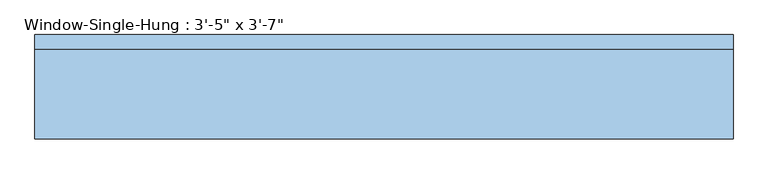
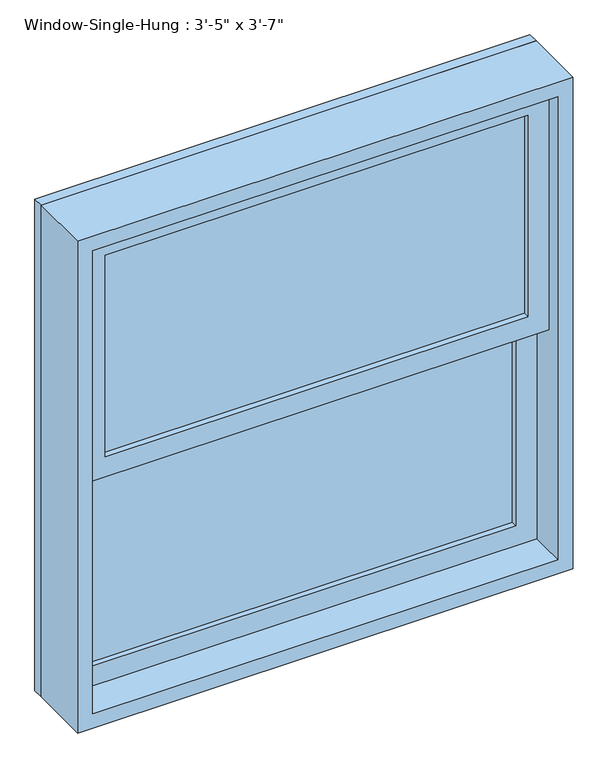
"""IFC4 building model written with IfcOpenShell, lengths in millimetres: window geometry."""

import ifcopenshell
import ifcopenshell.guid

model = None  # the IFC model being written
_history = None  # IfcOwnerHistory: only IFC2X3 demands one
_inside = {}  # id of a spatial element -> (the spatial element, [elements in it])
_under = {}  # id of a project, library or spatial element -> (it, [spatial elements below it])
_declared = {}  # id of a project -> (the project, [libraries it declares])
_typed = {}  # id of a type object -> (the type object, [elements of that type])
_made_of = {}  # id of a material, layer set ... -> (it, [elements and type objects made of it])


def new_model(schema):
    """Start an empty IFC model of exactly this schema.

    Asked for "IFC4X3", IfcOpenShell would pick the latest addendum, in which some entities
    have other attributes; the version numbers below select the first issue.
    IFC2X3 requires an IfcOwnerHistory on every rooted entity: one is made here for all.
    """
    global model, _history
    if schema == "IFC4X3":
        model = ifcopenshell.file(schema_version=(4, 3, 0, 0))
    else:
        model = ifcopenshell.file(schema=schema)
    _inside.clear()
    _under.clear()
    _declared.clear()
    _typed.clear()
    _made_of.clear()
    _history = None
    if model.schema == "IFC2X3":
        org = make("IfcOrganization", Name="unknown")
        user = make(
            "IfcPersonAndOrganization",
            ThePerson=make("IfcPerson", FamilyName="unknown"),
            TheOrganization=org,
        )
        app = make(
            "IfcApplication",
            ApplicationDeveloper=org,
            Version="unknown",
            ApplicationFullName="unknown",
            ApplicationIdentifier="unknown",
        )
        _history = make(
            "IfcOwnerHistory",
            OwningUser=user,
            OwningApplication=app,
            ChangeAction="ADDED",
            CreationDate=0,
        )
    return model


def make(cls, **values):
    """One entity of the class cls with the attributes given. An attribute that is None is left unset."""
    return model.create_entity(
        cls, **{name: value for name, value in values.items() if value is not None}
    )


def rooted(cls, **values):
    """An entity with a GlobalId (a new one), such as an element, a storey or a relation."""
    return make(cls, GlobalId=ifcopenshell.guid.new(), OwnerHistory=_history, **values)


def si_unit(unit_type, name, prefix=None):
    """IfcSIUnit, for example si_unit("LENGTHUNIT", "METRE", prefix="MILLI")."""
    return make("IfcSIUnit", UnitType=unit_type, Prefix=prefix, Name=name)


def assignment(units):
    """IfcUnitAssignment: the units of a project."""
    return None if units is None else make("IfcUnitAssignment", Units=units)


def point(xyz):
    """IfcCartesianPoint."""
    return None if xyz is None else make("IfcCartesianPoint", Coordinates=xyz)


def direction(xyz):
    """IfcDirection."""
    return None if xyz is None else make("IfcDirection", DirectionRatios=xyz)


def frame(location, z_axis=None, x_axis=None):
    """IfcAxis2Placement3D, a coordinate frame: its origin and axes. An axis left out is left unset."""
    return make(
        "IfcAxis2Placement3D",
        Location=point(location),
        Axis=direction(z_axis),
        RefDirection=direction(x_axis),
    )


def origin():
    """The frame at (0, 0, 0) with its axes left unset."""
    return frame((0.0, 0.0, 0.0))


def place(relative_to, where):
    """IfcLocalPlacement: puts the frame where relative to a parent placement (None: the world)."""
    return make(
        "IfcLocalPlacement", PlacementRelTo=relative_to, RelativePlacement=where
    )


def context(
    kind, dimensions, precision=None, world=None, true_north=None, identifier=None
):
    """IfcGeometricRepresentationContext, for example the 3D "Model" context."""
    return make(
        "IfcGeometricRepresentationContext",
        ContextIdentifier=identifier,
        ContextType=kind,
        CoordinateSpaceDimension=dimensions,
        Precision=precision,
        WorldCoordinateSystem=world,
        TrueNorth=true_north,
    )


def project(units=None, contexts=None):
    """IfcProject with its units and contexts."""
    return rooted(
        "IfcProject",
        Name="project",
        RepresentationContexts=contexts,
        UnitsInContext=assignment(units),
    )


def spatial(cls, under=None, at=None, **own):
    """A site, building, storey or space (cls), placed at a placement, below another one or the project."""
    s = rooted(cls, ObjectPlacement=at, **own)
    if under is not None:
        _under.setdefault(under.id(), (under, []))[1].append(s)
    return s


def polyline(points):
    """IfcPolyline through the points."""
    return make("IfcPolyline", Points=[point(p) for p in points])


def outline(outer, holes=None, kind="AREA"):
    """IfcArbitraryClosedProfileDef: a profile drawn as a closed curve; with holes, ...WithVoids."""
    if holes is None:
        return make("IfcArbitraryClosedProfileDef", ProfileType=kind, OuterCurve=outer)
    return make(
        "IfcArbitraryProfileDefWithVoids",
        ProfileType=kind,
        OuterCurve=outer,
        InnerCurves=holes,
    )


def extrude(swept, where, along, depth):
    """IfcExtrudedAreaSolid: the profile swept, set in the frame where, extruded along a direction by depth."""
    return make(
        "IfcExtrudedAreaSolid",
        SweptArea=swept,
        Position=where,
        ExtrudedDirection=direction(along),
        Depth=depth,
    )


def shape(context_of_items, identifier, shape_type, items):
    """IfcShapeRepresentation: the items that make up one representation, for example the "Body"."""
    return make(
        "IfcShapeRepresentation",
        ContextOfItems=context_of_items,
        RepresentationIdentifier=identifier,
        RepresentationType=shape_type,
        Items=items,
    )


def source(mapping_origin, context_of_items, identifier, shape_type, items):
    """IfcRepresentationMap: a shape defined once, which mapped items show again and again."""
    return make(
        "IfcRepresentationMap",
        MappingOrigin=mapping_origin,
        MappedRepresentation=shape(context_of_items, identifier, shape_type, items),
    )


def transform(
    local_origin,
    x_axis=None,
    y_axis=None,
    z_axis=None,
    scale=None,
    scale2=None,
    scale3=None,
    uniform=True,
):
    """IfcCartesianTransformationOperator3D, or its non-uniform kind. x_axis, y_axis, z_axis: its Axis1, 2, 3."""
    if uniform:
        return make(
            "IfcCartesianTransformationOperator3D",
            Axis1=direction(x_axis),
            Axis2=direction(y_axis),
            LocalOrigin=point(local_origin),
            Scale=scale,
            Axis3=direction(z_axis),
        )
    return make(
        "IfcCartesianTransformationOperator3DnonUniform",
        Axis1=direction(x_axis),
        Axis2=direction(y_axis),
        LocalOrigin=point(local_origin),
        Scale=scale,
        Axis3=direction(z_axis),
        Scale2=scale2,
        Scale3=scale3,
    )


def mapped(mapping_source, mapping_target):
    """IfcMappedItem: shows the shape of a source again, moved by a transform."""
    return make(
        "IfcMappedItem", MappingSource=mapping_source, MappingTarget=mapping_target
    )


def made_of(thing, what):
    """Note that an element or type object is made of a material, layer set ...; save() writes the relation."""
    if what is not None:
        _made_of.setdefault(what.id(), (what, []))[1].append(thing)
    return thing


def element(
    cls,
    number,
    at=None,
    inside=None,
    cuts=None,
    type_object=None,
    material=None,
    context=None,
    identifier="Body",
    shape_type=None,
    held_by="IfcProductDefinitionShape",
    body=None,
    shapes=None,
    **own,
):
    """One element of the class cls, such as IfcWall. Its Tag is "e" and its number.

    at: its placement. inside: the storey or other place that contains it. cuts: it is an
    opening in that element (IfcRelVoidsElement). A single representation is given by context,
    identifier, shape_type and body (its items); several are given by shapes. held_by: the class
    of the entity that holds the representations. save() writes the other relations.
    """
    e = rooted(cls, Tag="e%d" % number, ObjectPlacement=at, **own)
    if body is not None:
        shapes = [shape(context, identifier, shape_type, body)]
    if shapes is not None:
        e.Representation = make(held_by, Representations=shapes)
    if inside is not None:
        _inside.setdefault(inside.id(), (inside, []))[1].append(e)
    if cuts is not None:
        rooted(
            "IfcRelVoidsElement", RelatingBuildingElement=cuts, RelatedOpeningElement=e
        )
    if type_object is not None:
        _typed.setdefault(type_object.id(), (type_object, []))[1].append(e)
    return made_of(e, material)


def aggregate(whole, parts):
    """IfcRelAggregates: a whole, such as a stair, and the parts it consists of."""
    return rooted("IfcRelAggregates", RelatingObject=whole, RelatedObjects=parts)


def save(model, path):
    """Write the relations noted so far, then the file.

    IfcRelAggregates (storeys below a building ...), IfcRelContainedInSpatialStructure (elements
    in a storey), IfcRelDefinesByType, IfcRelAssociatesMaterial and IfcRelDeclares: one each for
    every whole, place, type object, material and project.
    """
    for whole, parts in _under.values():
        aggregate(whole, parts)
    for where, things in _inside.values():
        rooted(
            "IfcRelContainedInSpatialStructure",
            RelatedElements=things,
            RelatingStructure=where,
        )
    for kind, things in _typed.values():
        rooted("IfcRelDefinesByType", RelatedObjects=things, RelatingType=kind)
    for what, things in _made_of.values():
        rooted("IfcRelAssociatesMaterial", RelatedObjects=things, RelatingMaterial=what)
    for by, libraries in _declared.values():
        rooted("IfcRelDeclares", RelatingContext=by, RelatedDefinitions=libraries)
    model.write(path)


def window_8f49ead4(model_context):
    return source(origin(), model_context, "Body", "SweptSolid", [
        extrude(outline(polyline([(444.5, 1.5875), (-444.5, 1.5875), (-444.5, 7.9375), (444.5, 7.9375), (444.5, 1.5875)])), frame((0.0, 0.0, 990.6), z_axis=(0.0, 0.0, 1.0), x_axis=(1.0, 0.0, 0.0)), (0.0, 0.0, 1.0), 447.675),
        extrude(outline(polyline([(-444.5, 14.2875), (-444.5, 20.6375), (444.5, 20.6375), (444.5, 14.2875), (-444.5, 14.2875)])), frame((0.0, 0.0, 990.6), z_axis=(0.0, 0.0, 1.0), x_axis=(1.0, 0.0, 0.0)), (0.0, 0.0, 1.0), 447.675),
        extrude(outline(polyline([(444.5, -42.8625), (-444.5, -42.8625), (-444.5, -36.5125), (444.5, -36.5125), (444.5, -42.8625)])), frame((0.0, 0.0, 1482.725), z_axis=(0.0, 0.0, 1.0), x_axis=(1.0, 0.0, 0.0)), (0.0, 0.0, 1.0), 447.675),
        extrude(outline(polyline([(-444.5, -30.1625), (-444.5, -23.8125), (444.5, -23.8125), (444.5, -30.1625), (-444.5, -30.1625)])), frame((0.0, 0.0, 1482.725), z_axis=(0.0, 0.0, 1.0), x_axis=(1.0, 0.0, 0.0)), (0.0, 0.0, 1.0), 447.675),
        extrude(outline(polyline([(1482.725, 488.95), (1482.725, -488.95), (946.15, -488.95), (946.15, 488.95), (1482.725, 488.95)]), holes=[polyline([(1438.275, -444.5), (1438.275, 444.5), (990.6, 444.5), (990.6, -444.5), (1438.275, -444.5)])]), frame((0.0, -11.1125, 0.0), z_axis=(0.0, 1.0, 0.0), x_axis=(0.0, 0.0, 1.0)), (0.0, 0.0, 1.0), 44.45),
        extrude(outline(polyline([(1974.85, 488.95), (1974.85, -488.95), (1438.275, -488.95), (1438.275, 488.95), (1974.85, 488.95)]), holes=[polyline([(1930.4, -444.5), (1930.4, 444.5), (1482.725, 444.5), (1482.725, -444.5), (1930.4, -444.5)])]), frame((0.0, -55.5625, 0.0), z_axis=(0.0, 1.0, 0.0), x_axis=(0.0, 0.0, 1.0)), (0.0, 0.0, 1.0), 44.45),
        extrude(outline(polyline([(2006.6, 520.7), (2006.6, -520.7), (914.4, -520.7), (914.4, 520.7), (2006.6, 520.7)]), holes=[polyline([(1974.85, -488.95), (1974.85, 488.95), (946.15, 488.95), (946.15, -488.95), (1974.85, -488.95)])]), frame((0.0, -87.3125, 0.0), z_axis=(0.0, 1.0, 0.0), x_axis=(0.0, 0.0, 1.0)), (0.0, 0.0, 1.0), 133.35),
        extrude(outline(polyline([(2006.6, 520.7), (2006.6, -520.7), (914.4, -520.7), (914.4, 520.7), (2006.6, 520.7)]), holes=[polyline([(1987.55, 501.65), (933.45, 501.65), (933.45, -501.65), (1987.55, -501.65), (1987.55, 501.65)])]), frame((0.0, 46.0375, 0.0), z_axis=(0.0, 1.0, 0.0), x_axis=(0.0, 0.0, 1.0)), (0.0, 0.0, 1.0), 22.225),
    ])


if __name__ == "__main__":
    model = new_model("IFC4")
    model_context = context("Model", 3, world=origin())
    ifc_project = project(units=[si_unit("LENGTHUNIT", "METRE", prefix="MILLI")], contexts=[model_context])
    site = spatial("IfcSite", under=ifc_project)
    building = spatial("IfcBuilding", under=site)
    placement = place(None, origin())
    window_shape = window_8f49ead4(model_context)
    element("IfcWindow", 1, ObjectType="Window-Single-Hung : 3'-5\" x 3'-7\"", at=placement, inside=building, context=model_context, shape_type="MappedRepresentation", body=[
        mapped(window_shape, transform((0.0, 0.0, 0.0), x_axis=(1.0, 0.0, 0.0), y_axis=(0.0, 1.0, 0.0), z_axis=(0.0, 0.0, 1.0))),
    ])
    save(model, "model.ifc")

# Revit data of these elements
# Type "Window-Single-Hung : 3'-5\" x 3'-7\""
#   Type Mark = "25"
#   Fire Rating = "0.5h"
#   Construction Type Id = "DG-DR"
#   Assembly Code = "B2020100"
#   Analytic Construction = "Double glazing - domestic"
#   Wall Thickness [instance default] = 0' - 6"
#   Window Inset [instance default] = 0' - 0"
#   Visual Light Transmittance = 0.81
#   Thermal Resistance (R) = 0.319569 (m²·K)/W
#   Solar Heat Gain Coefficient = 0.76
#   Muntin Width = 2' - 11"
#   Muntin Height = 1' - 5 5/8"
#   Interior Wall Closure [instance default] = 0' - 1 1/2"
#   Rough Width = 3' - 5 1/2"
#   Rough Height = 3' - 7 1/2"
#   Frame Extension [instance default] = 0' - 1 1/4"
#   Exterior Wall Closure [instance default] = 0' - 0 1/2"
#   Extension Jamb [instance default] = 0' - 1 1/2"
#   Heat Transfer Coefficient (U) = 3.12929 W/(m²·K)
#   Height = 3' - 7"
#   Width = 3' - 5"
#   Top Muntin Visibility = yes
#   Indicator Visibility [instance default] = yes
#   Extension Jamb Visibility [instance default] = yes
#   Interior Trim Visibility [instance default] = yes
#   Exterior Trim Visibility [instance default] = yes
#   Bottom Muntin Visibility = yes
#   Muntin Pattern = Muntin Pattern_2x2 : Muntin Pattern_2x2
#   Interior Trim Material = Wood - Stained
#   Interior Trim = Trim-Window-Interior-Flat : Picture Frame
#   Exterior Trim Material = Clad - White
#   Exterior Trim = Trim-Window-Exterior-Flat : with Sill
#   Glass Panel Material = Glass
#   Exterior Frame Material = Clad - White
#   Interior Frame Material = Wood - Stained
#   Wall Closure = (empty or 0)
# Element 1 (IfcWindow, "Window-Single-Hung : 3'-5\" x 3'-7\"")
#   Wall Thickness = 0' - 5 3/8"
#   Extension Jamb = 0' - 0 7/8"
#   Materials on its faces: "Wood - Stained", "Glass", "Clad - White"
# Materials
#   "Wood - Stained": class "Wood", colour RGB 224 178 126, transparency 0, Cost = 0
#   "Clad - White": class "Wood", colour RGB 242 242 238, transparency 0, Cost = 0
#   "Glass": class "Glass", colour RGB 0 128 192, transparency 0.75, Description = "Soda Lime Glass", Cost = 0
